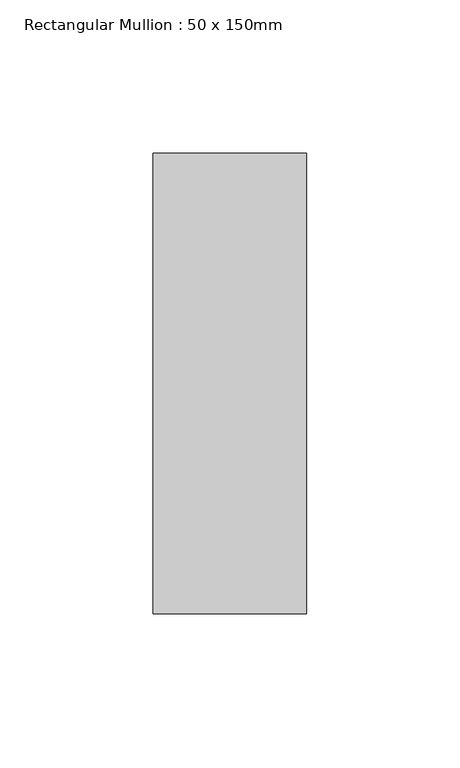
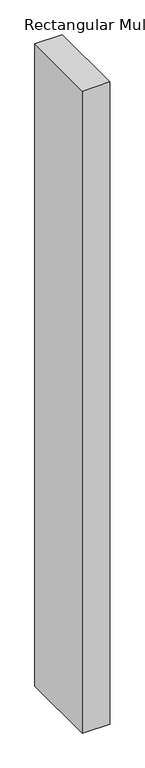
"""IFC4 building model written with IfcOpenShell, lengths in millimetres: member geometry, Rectangular Mullion : 50 x 150mm."""

from ifc_helpers import new_model, si_unit, frame, origin, place, context, project, spatial, polyline, outline, extrude, source, transform, mapped, element, save


def rectangular_mullion_50_x_150mm_c0f05268(model_context):
    return source(origin(), model_context, "Body", "SweptSolid", [
        extrude(outline(polyline([(25.0, 75.0), (25.0, -75.0), (-25.0, -75.0), (-25.0, 75.0), (25.0, 75.0)])), frame((0.0, 0.0, -1241.1082713), z_axis=(0.0, 0.0, 1.0), x_axis=(1.0, 0.0, 0.0)), (0.0, 0.0, 1.0), 1241.1082713),
    ])


if __name__ == "__main__":
    model = new_model("IFC4")
    model_context = context("Model", 3, world=origin())
    ifc_project = project(units=[si_unit("LENGTHUNIT", "METRE", prefix="MILLI")], contexts=[model_context])
    site = spatial("IfcSite", under=ifc_project)
    building = spatial("IfcBuilding", under=site)
    placement = place(None, origin())
    rectangular_mullion_50_x_150mm_shape = rectangular_mullion_50_x_150mm_c0f05268(model_context)
    element("IfcMember", 1, ObjectType="Rectangular Mullion : 50 x 150mm", at=placement, inside=building, context=model_context, shape_type="MappedRepresentation", body=[
        mapped(rectangular_mullion_50_x_150mm_shape, transform((0.0, 0.0, 0.0), x_axis=(1.0, 0.0, 0.0), y_axis=(0.0, 1.0, 0.0), z_axis=(0.0, 0.0, 1.0))),
    ])
    save(model, "model.ifc")

# Revit data of these elements
# Type "Rectangular Mullion : 50 x 150mm"
#   built-in parameter 1007304 = 0.492126 (stored number, unit not read)
#   built-in parameter 1007301 = 0.082021 (stored number, unit not read)
#   built-in parameter 1007300 = 0.082021 (stored number, unit not read)
# Element 1 (IfcMember, "Rectangular Mullion : 50 x 150mm")
#   Materials on its faces: "Aluminium"
# Materials
#   "Aluminium": class "Metal", colour RGB 247 247 247, transparency 0, Description = "Aluminium 6061", Cost = 0
